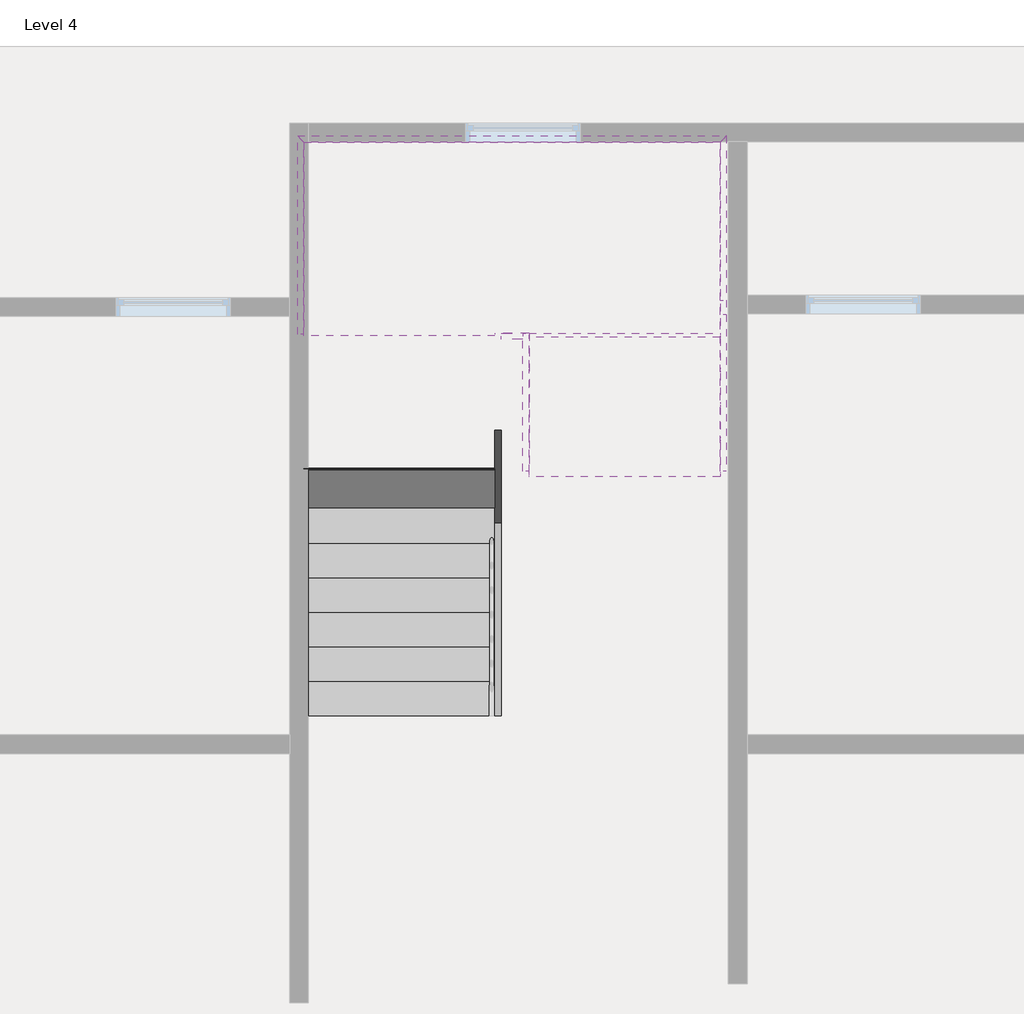
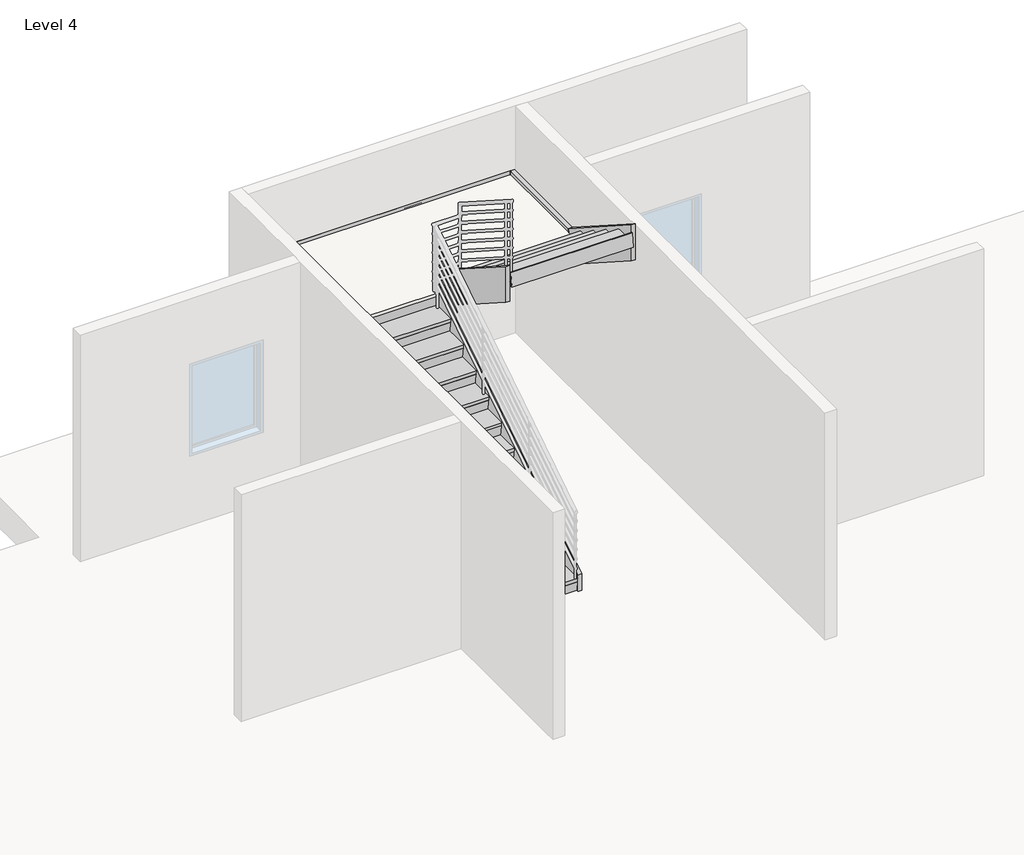
# One storey, part 7 of 7: 8 members, 2 stair flights, 1 slab.
"""IFC4 building model written with IfcOpenShell, lengths in millimetres."""

import ifcopenshell
import ifcopenshell.guid

model = None  # the IFC model being written
_history = None  # IfcOwnerHistory: only IFC2X3 demands one
_inside = {}  # id of a spatial element -> (the spatial element, [elements in it])
_under = {}  # id of a project, library or spatial element -> (it, [spatial elements below it])
_declared = {}  # id of a project -> (the project, [libraries it declares])
_typed = {}  # id of a type object -> (the type object, [elements of that type])
_made_of = {}  # id of a material, layer set ... -> (it, [elements and type objects made of it])


def new_model(schema):
    """Start an empty IFC model of exactly this schema.

    Asked for "IFC4X3", IfcOpenShell would pick the latest addendum, in which some entities
    have other attributes; the version numbers below select the first issue.
    IFC2X3 requires an IfcOwnerHistory on every rooted entity: one is made here for all.
    """
    global model, _history
    if schema == "IFC4X3":
        model = ifcopenshell.file(schema_version=(4, 3, 0, 0))
    else:
        model = ifcopenshell.file(schema=schema)
    _inside.clear()
    _under.clear()
    _declared.clear()
    _typed.clear()
    _made_of.clear()
    _history = None
    if model.schema == "IFC2X3":
        org = make("IfcOrganization", Name="unknown")
        user = make(
            "IfcPersonAndOrganization",
            ThePerson=make("IfcPerson", FamilyName="unknown"),
            TheOrganization=org,
        )
        app = make(
            "IfcApplication",
            ApplicationDeveloper=org,
            Version="unknown",
            ApplicationFullName="unknown",
            ApplicationIdentifier="unknown",
        )
        _history = make(
            "IfcOwnerHistory",
            OwningUser=user,
            OwningApplication=app,
            ChangeAction="ADDED",
            CreationDate=0,
        )
    return model


def make(cls, **values):
    """One entity of the class cls with the attributes given. An attribute that is None is left unset."""
    return model.create_entity(
        cls, **{name: value for name, value in values.items() if value is not None}
    )


def rooted(cls, **values):
    """An entity with a GlobalId (a new one), such as an element, a storey or a relation."""
    return make(cls, GlobalId=ifcopenshell.guid.new(), OwnerHistory=_history, **values)


def si_unit(unit_type, name, prefix=None):
    """IfcSIUnit, for example si_unit("LENGTHUNIT", "METRE", prefix="MILLI")."""
    return make("IfcSIUnit", UnitType=unit_type, Prefix=prefix, Name=name)


def assignment(units):
    """IfcUnitAssignment: the units of a project."""
    return None if units is None else make("IfcUnitAssignment", Units=units)


def point(xyz):
    """IfcCartesianPoint."""
    return None if xyz is None else make("IfcCartesianPoint", Coordinates=xyz)


def direction(xyz):
    """IfcDirection."""
    return None if xyz is None else make("IfcDirection", DirectionRatios=xyz)


def frame(location, z_axis=None, x_axis=None):
    """IfcAxis2Placement3D, a coordinate frame: its origin and axes. An axis left out is left unset."""
    return make(
        "IfcAxis2Placement3D",
        Location=point(location),
        Axis=direction(z_axis),
        RefDirection=direction(x_axis),
    )


def origin():
    """The frame at (0, 0, 0) with its axes left unset."""
    return frame((0.0, 0.0, 0.0))


def place(relative_to, where):
    """IfcLocalPlacement: puts the frame where relative to a parent placement (None: the world)."""
    return make(
        "IfcLocalPlacement", PlacementRelTo=relative_to, RelativePlacement=where
    )


def context(
    kind, dimensions, precision=None, world=None, true_north=None, identifier=None
):
    """IfcGeometricRepresentationContext, for example the 3D "Model" context."""
    return make(
        "IfcGeometricRepresentationContext",
        ContextIdentifier=identifier,
        ContextType=kind,
        CoordinateSpaceDimension=dimensions,
        Precision=precision,
        WorldCoordinateSystem=world,
        TrueNorth=true_north,
    )


def project(units=None, contexts=None):
    """IfcProject with its units and contexts."""
    return rooted(
        "IfcProject",
        Name="project",
        RepresentationContexts=contexts,
        UnitsInContext=assignment(units),
    )


def spatial(cls, under=None, at=None, **own):
    """A site, building, storey or space (cls), placed at a placement, below another one or the project."""
    s = rooted(cls, ObjectPlacement=at, **own)
    if under is not None:
        _under.setdefault(under.id(), (under, []))[1].append(s)
    return s


def polyline(points):
    """IfcPolyline through the points."""
    return make("IfcPolyline", Points=[point(p) for p in points])


def outline(outer, holes=None, kind="AREA"):
    """IfcArbitraryClosedProfileDef: a profile drawn as a closed curve; with holes, ...WithVoids."""
    if holes is None:
        return make("IfcArbitraryClosedProfileDef", ProfileType=kind, OuterCurve=outer)
    return make(
        "IfcArbitraryProfileDefWithVoids",
        ProfileType=kind,
        OuterCurve=outer,
        InnerCurves=holes,
    )


def extrude(swept, where, along, depth):
    """IfcExtrudedAreaSolid: the profile swept, set in the frame where, extruded along a direction by depth."""
    return make(
        "IfcExtrudedAreaSolid",
        SweptArea=swept,
        Position=where,
        ExtrudedDirection=direction(along),
        Depth=depth,
    )


def faces_of(points, faces, orient=None, outer=None):
    """IfcFace entities. A face is a list of loops; a loop is a list of indices into points, from 0.

    orient and outer hold one flag for each loop. By default every Orientation is true, the
    first loop of a face is its IfcFaceOuterBound and the others are IfcFaceBound.
    """
    made = []
    for i, loops in enumerate(faces):
        bounds = []
        for j, loop in enumerate(loops):
            is_outer = j == 0 if outer is None else outer[i][j]
            bounds.append(
                make(
                    "IfcFaceOuterBound" if is_outer else "IfcFaceBound",
                    Bound=make("IfcPolyLoop", Polygon=[points[k] for k in loop]),
                    Orientation=True if orient is None else orient[i][j],
                )
            )
        made.append(make("IfcFace", Bounds=bounds))
    return made


def faceted_brep(points, faces, orient=None, outer=None, voids=None):
    """IfcFacetedBrep: a solid bounded by flat faces; with voids (closed shells), ...WithVoids."""
    shared = [point(p) for p in points]
    hull = make("IfcClosedShell", CfsFaces=faces_of(shared, faces, orient, outer))
    if voids is None:
        return make("IfcFacetedBrep", Outer=hull)
    return make(
        "IfcFacetedBrepWithVoids",
        Outer=hull,
        Voids=[
            make(cls, CfsFaces=faces_of(shared, fs, o, b)) for cls, fs, o, b in voids
        ],
    )


def shape(context_of_items, identifier, shape_type, items):
    """IfcShapeRepresentation: the items that make up one representation, for example the "Body"."""
    return make(
        "IfcShapeRepresentation",
        ContextOfItems=context_of_items,
        RepresentationIdentifier=identifier,
        RepresentationType=shape_type,
        Items=items,
    )


def source(mapping_origin, context_of_items, identifier, shape_type, items):
    """IfcRepresentationMap: a shape defined once, which mapped items show again and again."""
    return make(
        "IfcRepresentationMap",
        MappingOrigin=mapping_origin,
        MappedRepresentation=shape(context_of_items, identifier, shape_type, items),
    )


def transform(
    local_origin,
    x_axis=None,
    y_axis=None,
    z_axis=None,
    scale=None,
    scale2=None,
    scale3=None,
    uniform=True,
):
    """IfcCartesianTransformationOperator3D, or its non-uniform kind. x_axis, y_axis, z_axis: its Axis1, 2, 3."""
    if uniform:
        return make(
            "IfcCartesianTransformationOperator3D",
            Axis1=direction(x_axis),
            Axis2=direction(y_axis),
            LocalOrigin=point(local_origin),
            Scale=scale,
            Axis3=direction(z_axis),
        )
    return make(
        "IfcCartesianTransformationOperator3DnonUniform",
        Axis1=direction(x_axis),
        Axis2=direction(y_axis),
        LocalOrigin=point(local_origin),
        Scale=scale,
        Axis3=direction(z_axis),
        Scale2=scale2,
        Scale3=scale3,
    )


def mapped(mapping_source, mapping_target):
    """IfcMappedItem: shows the shape of a source again, moved by a transform."""
    return make(
        "IfcMappedItem", MappingSource=mapping_source, MappingTarget=mapping_target
    )


def made_of(thing, what):
    """Note that an element or type object is made of a material, layer set ...; save() writes the relation."""
    if what is not None:
        _made_of.setdefault(what.id(), (what, []))[1].append(thing)
    return thing


def element(
    cls,
    number,
    at=None,
    inside=None,
    cuts=None,
    type_object=None,
    material=None,
    context=None,
    identifier="Body",
    shape_type=None,
    held_by="IfcProductDefinitionShape",
    body=None,
    shapes=None,
    **own,
):
    """One element of the class cls, such as IfcWall. Its Tag is "e" and its number.

    at: its placement. inside: the storey or other place that contains it. cuts: it is an
    opening in that element (IfcRelVoidsElement). A single representation is given by context,
    identifier, shape_type and body (its items); several are given by shapes. held_by: the class
    of the entity that holds the representations. save() writes the other relations.
    """
    e = rooted(cls, Tag="e%d" % number, ObjectPlacement=at, **own)
    if body is not None:
        shapes = [shape(context, identifier, shape_type, body)]
    if shapes is not None:
        e.Representation = make(held_by, Representations=shapes)
    if inside is not None:
        _inside.setdefault(inside.id(), (inside, []))[1].append(e)
    if cuts is not None:
        rooted(
            "IfcRelVoidsElement", RelatingBuildingElement=cuts, RelatedOpeningElement=e
        )
    if type_object is not None:
        _typed.setdefault(type_object.id(), (type_object, []))[1].append(e)
    return made_of(e, material)


def aggregate(whole, parts):
    """IfcRelAggregates: a whole, such as a stair, and the parts it consists of."""
    return rooted("IfcRelAggregates", RelatingObject=whole, RelatedObjects=parts)


def save(model, path):
    """Write the relations noted so far, then the file.

    IfcRelAggregates (storeys below a building ...), IfcRelContainedInSpatialStructure (elements
    in a storey), IfcRelDefinesByType, IfcRelAssociatesMaterial and IfcRelDeclares: one each for
    every whole, place, type object, material and project.
    """
    for whole, parts in _under.values():
        aggregate(whole, parts)
    for where, things in _inside.values():
        rooted(
            "IfcRelContainedInSpatialStructure",
            RelatedElements=things,
            RelatingStructure=where,
        )
    for kind, things in _typed.values():
        rooted("IfcRelDefinesByType", RelatedObjects=things, RelatingType=kind)
    for what, things in _made_of.values():
        rooted("IfcRelAssociatesMaterial", RelatedObjects=things, RelatingMaterial=what)
    for by, libraries in _declared.values():
        rooted("IfcRelDeclares", RelatingContext=by, RelatedDefinitions=libraries)
    model.write(path)


def non_monolithic_landing_893569eb(model_context):
    return source(origin(), model_context, "Body", "Brep", [
        faceted_brep([(-226.7120949, 7307.4781803, 11617.6470588), (-226.7120949, 7300.3948469, 11567.6470588), (1293.2879051, 7300.3948469, 11567.6470588), (1293.2879051, 7307.4781803, 11617.6470588), (-499.4393676, 7309.7509075, 11617.6470588), (-499.4393676, 7332.4781803, 11617.6470588), (-226.7120949, 7332.4781803, 11617.6470588), (1293.2879051, 7332.4781803, 11617.6470588), (1293.2879051, 8852.4781803, 11617.6470588), (-2019.4393676, 8852.4781803, 11617.6470588), (-2019.4393676, 7309.7509075, 11617.6470588), (-226.7120949, 7332.4781803, 11567.6470588), (-499.4393676, 7332.4781803, 11567.6470588), (-499.4393676, 7316.8342409, 11567.6470588), (-2019.4393676, 7316.8342409, 11567.6470588), (-2019.4393676, 8852.4781803, 11567.6470588), (1293.2879051, 8852.4781803, 11567.6470588), (1293.2879051, 7332.4781803, 11567.6470588)], [[[0, 1, 2, 3]], [[4, 5, 6, 0, 3, 7, 8, 9, 10]], [[11, 12, 13, 14, 15, 16, 17, 2, 1]], [[5, 4, 13, 12]], [[6, 5, 12, 11]], [[0, 6, 11, 1]], [[7, 3, 2, 17]], [[8, 7, 17, 16]], [[9, 8, 16, 15]], [[10, 9, 15, 14]], [[4, 10, 14, 13]]]),
    ])


def stair_flight_50mm_tread_25mm_nosing_13mm_riser_ea8afa7a(model_context):
    return source(origin(), model_context, "Body", "Brep", [
        faceted_brep([(-499.4393676, 4584.7509075, 9676.4705882), (-499.4393676, 4591.8342409, 9626.4705882), (-2019.4393676, 4591.8342409, 9626.4705882), (-2019.4393676, 4584.7509075, 9676.4705882), (-2019.4393676, 4284.7509075, 9676.4705882), (-499.4393676, 4284.7509075, 9676.4705882), (-499.4393676, 4291.8342409, 9626.4705882), (-2019.4393676, 4291.8342409, 9626.4705882)], [[[0, 1, 2, 3]], [[3, 4, 5, 0]], [[2, 1, 6, 7]], [[4, 3, 2, 7]], [[0, 5, 6, 1]], [[5, 4, 7, 6]]]),
        faceted_brep([(-499.4393676, 4291.8342409, 9626.4705882), (-499.4393676, 4309.7509075, 9500.0), (-499.4393676, 4322.3757185, 9500.0), (-499.4393676, 4304.4590518, 9626.4705882), (-2019.4393676, 4291.8342409, 9626.4705882), (-2019.4393676, 4304.4590518, 9626.4705882), (-2019.4393676, 4322.3757185, 9500.0), (-2019.4393676, 4309.7509075, 9500.0)], [[[0, 1, 2, 3]], [[4, 5, 6, 7]], [[1, 0, 4, 7]], [[2, 1, 7, 6]], [[3, 2, 6, 5]], [[0, 3, 5, 4]]]),
        faceted_brep([(-499.4393676, 4566.8342409, 9802.9411765), (-499.4393676, 4591.8342409, 9626.4705882), (-499.4393676, 4604.4590518, 9626.4705882), (-499.4393676, 4579.4590518, 9802.9411765), (-2019.4393676, 4566.8342409, 9802.9411765), (-2019.4393676, 4579.4590518, 9802.9411765), (-2019.4393676, 4604.4590518, 9626.4705882), (-2019.4393676, 4591.8342409, 9626.4705882)], [[[0, 1, 2, 3]], [[4, 5, 6, 7]], [[1, 0, 4, 7]], [[2, 1, 7, 6]], [[3, 2, 6, 5]], [[0, 3, 5, 4]]]),
        faceted_brep([(-2019.4393676, 4859.7509075, 9852.9411765), (-2019.4393676, 4559.7509075, 9852.9411765), (-499.4393676, 4559.7509075, 9852.9411765), (-499.4393676, 4859.7509075, 9852.9411765), (-2019.4393676, 4866.8342409, 9802.9411765), (-499.4393676, 4866.8342409, 9802.9411765), (-499.4393676, 4566.8342409, 9802.9411765), (-2019.4393676, 4566.8342409, 9802.9411765)], [[[0, 1, 2, 3]], [[4, 5, 6, 7]], [[1, 0, 4, 7]], [[3, 2, 6, 5]], [[3, 5, 4, 0]], [[2, 1, 7, 6]]]),
        faceted_brep([(-499.4393676, 4841.8342409, 9979.4117647), (-499.4393676, 4866.8342409, 9802.9411765), (-499.4393676, 4879.4590518, 9802.9411765), (-499.4393676, 4854.4590518, 9979.4117647), (-2019.4393676, 4841.8342409, 9979.4117647), (-2019.4393676, 4854.4590518, 9979.4117647), (-2019.4393676, 4879.4590518, 9802.9411765), (-2019.4393676, 4866.8342409, 9802.9411765)], [[[0, 1, 2, 3]], [[4, 5, 6, 7]], [[1, 0, 4, 7]], [[2, 1, 7, 6]], [[3, 2, 6, 5]], [[0, 3, 5, 4]]]),
        faceted_brep([(-2019.4393676, 5134.7509075, 10029.4117647), (-2019.4393676, 4834.7509075, 10029.4117647), (-499.4393676, 4834.7509075, 10029.4117647), (-499.4393676, 5134.7509075, 10029.4117647), (-2019.4393676, 5141.8342409, 9979.4117647), (-499.4393676, 5141.8342409, 9979.4117647), (-499.4393676, 4841.8342409, 9979.4117647), (-2019.4393676, 4841.8342409, 9979.4117647)], [[[0, 1, 2, 3]], [[4, 5, 6, 7]], [[1, 0, 4, 7]], [[3, 2, 6, 5]], [[3, 5, 4, 0]], [[2, 1, 7, 6]]]),
        faceted_brep([(-499.4393676, 5116.8342409, 10155.8823529), (-499.4393676, 5141.8342409, 9979.4117647), (-499.4393676, 5154.4590518, 9979.4117647), (-499.4393676, 5129.4590518, 10155.8823529), (-2019.4393676, 5116.8342409, 10155.8823529), (-2019.4393676, 5129.4590518, 10155.8823529), (-2019.4393676, 5154.4590518, 9979.4117647), (-2019.4393676, 5141.8342409, 9979.4117647)], [[[0, 1, 2, 3]], [[4, 5, 6, 7]], [[1, 0, 4, 7]], [[2, 1, 7, 6]], [[3, 2, 6, 5]], [[0, 3, 5, 4]]]),
        faceted_brep([(-2019.4393676, 5409.7509075, 10205.8823529), (-2019.4393676, 5109.7509075, 10205.8823529), (-499.4393676, 5109.7509075, 10205.8823529), (-499.4393676, 5409.7509075, 10205.8823529), (-2019.4393676, 5416.8342409, 10155.8823529), (-499.4393676, 5416.8342409, 10155.8823529), (-499.4393676, 5116.8342409, 10155.8823529), (-2019.4393676, 5116.8342409, 10155.8823529)], [[[0, 1, 2, 3]], [[4, 5, 6, 7]], [[1, 0, 4, 7]], [[3, 2, 6, 5]], [[3, 5, 4, 0]], [[2, 1, 7, 6]]]),
        faceted_brep([(-499.4393676, 5391.8342409, 10332.3529412), (-499.4393676, 5416.8342409, 10155.8823529), (-499.4393676, 5429.4590518, 10155.8823529), (-499.4393676, 5404.4590518, 10332.3529412), (-2019.4393676, 5391.8342409, 10332.3529412), (-2019.4393676, 5404.4590518, 10332.3529412), (-2019.4393676, 5429.4590518, 10155.8823529), (-2019.4393676, 5416.8342409, 10155.8823529)], [[[0, 1, 2, 3]], [[4, 5, 6, 7]], [[1, 0, 4, 7]], [[2, 1, 7, 6]], [[3, 2, 6, 5]], [[0, 3, 5, 4]]]),
        faceted_brep([(-2019.4393676, 5684.7509075, 10382.3529412), (-2019.4393676, 5384.7509075, 10382.3529412), (-499.4393676, 5384.7509075, 10382.3529412), (-499.4393676, 5684.7509075, 10382.3529412), (-2019.4393676, 5691.8342409, 10332.3529412), (-499.4393676, 5691.8342409, 10332.3529412), (-499.4393676, 5391.8342409, 10332.3529412), (-2019.4393676, 5391.8342409, 10332.3529412)], [[[0, 1, 2, 3]], [[4, 5, 6, 7]], [[1, 0, 4, 7]], [[3, 2, 6, 5]], [[3, 5, 4, 0]], [[2, 1, 7, 6]]]),
        faceted_brep([(-499.4393676, 5666.8342409, 10508.8235294), (-499.4393676, 5691.8342409, 10332.3529412), (-499.4393676, 5704.4590518, 10332.3529412), (-499.4393676, 5679.4590518, 10508.8235294), (-2019.4393676, 5666.8342409, 10508.8235294), (-2019.4393676, 5679.4590518, 10508.8235294), (-2019.4393676, 5704.4590518, 10332.3529412), (-2019.4393676, 5691.8342409, 10332.3529412)], [[[0, 1, 2, 3]], [[4, 5, 6, 7]], [[1, 0, 4, 7]], [[2, 1, 7, 6]], [[3, 2, 6, 5]], [[0, 3, 5, 4]]]),
        faceted_brep([(-2019.4393676, 5959.7509075, 10558.8235294), (-2019.4393676, 5659.7509075, 10558.8235294), (-499.4393676, 5659.7509075, 10558.8235294), (-499.4393676, 5959.7509075, 10558.8235294), (-2019.4393676, 5966.8342409, 10508.8235294), (-499.4393676, 5966.8342409, 10508.8235294), (-499.4393676, 5666.8342409, 10508.8235294), (-2019.4393676, 5666.8342409, 10508.8235294)], [[[0, 1, 2, 3]], [[4, 5, 6, 7]], [[1, 0, 4, 7]], [[3, 2, 6, 5]], [[3, 5, 4, 0]], [[2, 1, 7, 6]]]),
        faceted_brep([(-499.4393676, 5941.8342409, 10685.2941176), (-499.4393676, 5966.8342409, 10508.8235294), (-499.4393676, 5979.4590518, 10508.8235294), (-499.4393676, 5954.4590518, 10685.2941176), (-2019.4393676, 5941.8342409, 10685.2941176), (-2019.4393676, 5954.4590518, 10685.2941176), (-2019.4393676, 5979.4590518, 10508.8235294), (-2019.4393676, 5966.8342409, 10508.8235294)], [[[0, 1, 2, 3]], [[4, 5, 6, 7]], [[1, 0, 4, 7]], [[2, 1, 7, 6]], [[3, 2, 6, 5]], [[0, 3, 5, 4]]]),
        faceted_brep([(-2019.4393676, 6234.7509075, 10735.2941176), (-2019.4393676, 5934.7509075, 10735.2941176), (-499.4393676, 5934.7509075, 10735.2941176), (-499.4393676, 6234.7509075, 10735.2941176), (-2019.4393676, 6241.8342409, 10685.2941176), (-499.4393676, 6241.8342409, 10685.2941176), (-499.4393676, 5941.8342409, 10685.2941176), (-2019.4393676, 5941.8342409, 10685.2941176)], [[[0, 1, 2, 3]], [[4, 5, 6, 7]], [[1, 0, 4, 7]], [[3, 2, 6, 5]], [[3, 5, 4, 0]], [[2, 1, 7, 6]]]),
        faceted_brep([(-499.4393676, 6216.8342409, 10861.7647059), (-499.4393676, 6241.8342409, 10685.2941176), (-499.4393676, 6254.4590518, 10685.2941176), (-499.4393676, 6229.4590518, 10861.7647059), (-2019.4393676, 6216.8342409, 10861.7647059), (-2019.4393676, 6229.4590518, 10861.7647059), (-2019.4393676, 6254.4590518, 10685.2941176), (-2019.4393676, 6241.8342409, 10685.2941176)], [[[0, 1, 2, 3]], [[4, 5, 6, 7]], [[1, 0, 4, 7]], [[2, 1, 7, 6]], [[3, 2, 6, 5]], [[0, 3, 5, 4]]]),
        faceted_brep([(-2019.4393676, 6509.7509075, 10911.7647059), (-2019.4393676, 6209.7509075, 10911.7647059), (-499.4393676, 6209.7509075, 10911.7647059), (-499.4393676, 6509.7509075, 10911.7647059), (-2019.4393676, 6516.8342409, 10861.7647059), (-499.4393676, 6516.8342409, 10861.7647059), (-499.4393676, 6216.8342409, 10861.7647059), (-2019.4393676, 6216.8342409, 10861.7647059)], [[[0, 1, 2, 3]], [[4, 5, 6, 7]], [[1, 0, 4, 7]], [[3, 2, 6, 5]], [[3, 5, 4, 0]], [[2, 1, 7, 6]]]),
        faceted_brep([(-499.4393676, 6491.8342409, 11038.2352941), (-499.4393676, 6516.8342409, 10861.7647059), (-499.4393676, 6529.4590518, 10861.7647059), (-499.4393676, 6504.4590518, 11038.2352941), (-2019.4393676, 6491.8342409, 11038.2352941), (-2019.4393676, 6504.4590518, 11038.2352941), (-2019.4393676, 6529.4590518, 10861.7647059), (-2019.4393676, 6516.8342409, 10861.7647059)], [[[0, 1, 2, 3]], [[4, 5, 6, 7]], [[1, 0, 4, 7]], [[2, 1, 7, 6]], [[3, 2, 6, 5]], [[0, 3, 5, 4]]]),
        faceted_brep([(-2019.4393676, 6784.7509075, 11088.2352941), (-2019.4393676, 6484.7509075, 11088.2352941), (-499.4393676, 6484.7509075, 11088.2352941), (-499.4393676, 6784.7509075, 11088.2352941), (-2019.4393676, 6791.8342409, 11038.2352941), (-499.4393676, 6791.8342409, 11038.2352941), (-499.4393676, 6491.8342409, 11038.2352941), (-2019.4393676, 6491.8342409, 11038.2352941)], [[[0, 1, 2, 3]], [[4, 5, 6, 7]], [[1, 0, 4, 7]], [[3, 2, 6, 5]], [[3, 5, 4, 0]], [[2, 1, 7, 6]]]),
        faceted_brep([(-499.4393676, 6766.8342409, 11214.7058824), (-499.4393676, 6791.8342409, 11038.2352941), (-499.4393676, 6804.4590518, 11038.2352941), (-499.4393676, 6779.4590518, 11214.7058824), (-2019.4393676, 6766.8342409, 11214.7058824), (-2019.4393676, 6779.4590518, 11214.7058824), (-2019.4393676, 6804.4590518, 11038.2352941), (-2019.4393676, 6791.8342409, 11038.2352941)], [[[0, 1, 2, 3]], [[4, 5, 6, 7]], [[1, 0, 4, 7]], [[2, 1, 7, 6]], [[3, 2, 6, 5]], [[0, 3, 5, 4]]]),
        faceted_brep([(-2019.4393676, 7059.7509075, 11264.7058824), (-2019.4393676, 6759.7509075, 11264.7058824), (-499.4393676, 6759.7509075, 11264.7058824), (-499.4393676, 7059.7509075, 11264.7058824), (-2019.4393676, 7066.8342409, 11214.7058824), (-499.4393676, 7066.8342409, 11214.7058824), (-499.4393676, 6766.8342409, 11214.7058824), (-2019.4393676, 6766.8342409, 11214.7058824)], [[[0, 1, 2, 3]], [[4, 5, 6, 7]], [[1, 0, 4, 7]], [[3, 2, 6, 5]], [[3, 5, 4, 0]], [[2, 1, 7, 6]]]),
        faceted_brep([(-499.4393676, 7316.8342409, 11567.6470588), (-499.4393676, 7341.8342409, 11391.1764706), (-499.4393676, 7354.4590518, 11391.1764706), (-499.4393676, 7329.4590518, 11567.6470588), (-2019.4393676, 7316.8342409, 11567.6470588), (-2019.4393676, 7329.4590518, 11567.6470588), (-2019.4393676, 7354.4590518, 11391.1764706), (-2019.4393676, 7341.8342409, 11391.1764706)], [[[0, 1, 2, 3]], [[4, 5, 6, 7]], [[1, 0, 4, 7]], [[2, 1, 7, 6]], [[3, 2, 6, 5]], [[0, 3, 5, 4]]]),
        faceted_brep([(-499.4393676, 7041.8342409, 11391.1764706), (-499.4393676, 7066.8342409, 11214.7058824), (-499.4393676, 7079.4590518, 11214.7058824), (-499.4393676, 7054.4590518, 11391.1764706), (-2019.4393676, 7041.8342409, 11391.1764706), (-2019.4393676, 7054.4590518, 11391.1764706), (-2019.4393676, 7079.4590518, 11214.7058824), (-2019.4393676, 7066.8342409, 11214.7058824)], [[[0, 1, 2, 3]], [[4, 5, 6, 7]], [[1, 0, 4, 7]], [[2, 1, 7, 6]], [[3, 2, 6, 5]], [[0, 3, 5, 4]]]),
        faceted_brep([(-2019.4393676, 7334.7509075, 11441.1764706), (-2019.4393676, 7309.7509075, 11441.1764706), (-2019.4393676, 7034.7509075, 11441.1764706), (-499.4393676, 7034.7509075, 11441.1764706), (-499.4393676, 7334.7509075, 11441.1764706), (-2019.4393676, 7341.8342409, 11391.1764706), (-499.4393676, 7341.8342409, 11391.1764706), (-499.4393676, 7041.8342409, 11391.1764706), (-2019.4393676, 7041.8342409, 11391.1764706), (-2019.4393676, 7309.7509075, 11391.1764706)], [[[0, 1, 2, 3, 4]], [[5, 6, 7, 8, 9]], [[1, 0, 5, 9]], [[2, 1, 9, 8]], [[4, 3, 7, 6]], [[4, 6, 5, 0]], [[3, 2, 8, 7]]]),
    ])


def stair_flight_50mm_tread_25mm_nosing_13mm_riser_c8de7c0f(model_context):
    return source(origin(), model_context, "Body", "SweptSolid", [
        extrude(outline(polyline([(7032.4781803, 11794.1176471), (7332.4781803, 11794.1176471), (7325.3948469, 11744.1176471), (7025.3948469, 11744.1176471), (7032.4781803, 11794.1176471)])), frame((-226.7120949, 0.0, 0.0), z_axis=(1.0, 0.0, 0.0), x_axis=(0.0, 1.0, 0.0)), (0.0, 0.0, 1.0), 1520.0),
        extrude(outline(polyline([(7325.3948469, 11744.1176471), (7300.3948469, 11567.6470588), (7287.770036, 11567.6470588), (7312.770036, 11744.1176471), (7325.3948469, 11744.1176471)])), frame((-226.7120949, 0.0, 0.0), z_axis=(1.0, 0.0, 0.0), x_axis=(0.0, 1.0, 0.0)), (0.0, 0.0, 1.0), 1520.0),
        extrude(outline(polyline([(7050.3948469, 11920.5882353), (7025.3948469, 11744.1176471), (7012.770036, 11744.1176471), (7037.770036, 11920.5882353), (7050.3948469, 11920.5882353)])), frame((-226.7120949, 0.0, 0.0), z_axis=(1.0, 0.0, 0.0), x_axis=(0.0, 1.0, 0.0)), (0.0, 0.0, 1.0), 1520.0),
        extrude(outline(polyline([(6757.4781803, 11970.5882353), (7057.4781803, 11970.5882353), (7050.3948469, 11920.5882353), (6750.3948469, 11920.5882353), (6757.4781803, 11970.5882353)])), frame((-226.7120949, 0.0, 0.0), z_axis=(1.0, 0.0, 0.0), x_axis=(0.0, 1.0, 0.0)), (0.0, 0.0, 1.0), 1520.0),
        extrude(outline(polyline([(6775.3948469, 12097.0588235), (6750.3948469, 11920.5882353), (6737.770036, 11920.5882353), (6762.770036, 12097.0588235), (6775.3948469, 12097.0588235)])), frame((-226.7120949, 0.0, 0.0), z_axis=(1.0, 0.0, 0.0), x_axis=(0.0, 1.0, 0.0)), (0.0, 0.0, 1.0), 1520.0),
        extrude(outline(polyline([(6482.4781803, 12147.0588235), (6782.4781803, 12147.0588235), (6775.3948469, 12097.0588235), (6475.3948469, 12097.0588235), (6482.4781803, 12147.0588235)])), frame((-226.7120949, 0.0, 0.0), z_axis=(1.0, 0.0, 0.0), x_axis=(0.0, 1.0, 0.0)), (0.0, 0.0, 1.0), 1520.0),
        extrude(outline(polyline([(6500.3948469, 12273.5294118), (6475.3948469, 12097.0588235), (6462.770036, 12097.0588235), (6487.770036, 12273.5294118), (6500.3948469, 12273.5294118)])), frame((-226.7120949, 0.0, 0.0), z_axis=(1.0, 0.0, 0.0), x_axis=(0.0, 1.0, 0.0)), (0.0, 0.0, 1.0), 1520.0),
        extrude(outline(polyline([(6225.3948469, 12450.0), (6200.3948469, 12273.5294118), (6187.770036, 12273.5294118), (6212.770036, 12450.0), (6225.3948469, 12450.0)])), frame((-226.7120949, 0.0, 0.0), z_axis=(1.0, 0.0, 0.0), x_axis=(0.0, 1.0, 0.0)), (0.0, 0.0, 1.0), 1520.0),
        extrude(outline(polyline([(6207.4781803, 12323.5294118), (6507.4781803, 12323.5294118), (6500.3948469, 12273.5294118), (6200.3948469, 12273.5294118), (6207.4781803, 12323.5294118)])), frame((-226.7120949, 0.0, 0.0), z_axis=(1.0, 0.0, 0.0), x_axis=(0.0, 1.0, 0.0)), (0.0, 0.0, 1.0), 1520.0),
    ])


model = new_model("IFC4")

# Units and contexts
model_context = context("Model", 3, world=origin())
ifc_project = project(units=[si_unit("LENGTHUNIT", "METRE", prefix="MILLI")], contexts=[model_context])

# Site, building, storey
site = spatial("IfcSite", under=ifc_project)
building = spatial("IfcBuilding", under=site)
storey = spatial("IfcBuildingStorey", under=building, Name="Level 4", Elevation=9500.0)

# Members
placement = place(None, origin())
element("IfcMember", 1, ObjectType="Stringer - 50mm Width", at=placement, inside=storey, context=model_context, shape_type="SweptSolid", body=[
    extrude(outline(polyline([(4284.7509075, 9500.0), (4284.7509075, 9715.9811749), (7322.0354678, 11665.0407858), (7439.3399977, 11265.0407858), (4688.8181065, 9500.0), (4284.7509075, 9500.0)])), frame((-2069.4393676, 0.0, 0.0), z_axis=(1.0, 0.0, 0.0), x_axis=(0.0, 1.0, 0.0)), (0.0, 0.0, 1.0), 50.0),
])
element("IfcMember", 2, ObjectType="Stringer - 50mm Width", at=placement, inside=storey, context=model_context, shape_type="SweptSolid", body=[
    extrude(outline(polyline([(4284.7509075, 9500.0), (4284.7509075, 9715.9811749), (7322.0354678, 11665.0407858), (7332.4781803, 11665.0407858), (7332.4781803, 11196.4663575), (4688.8181065, 9500.0), (4284.7509075, 9500.0)])), frame((-499.4393676, 0.0, 0.0), z_axis=(1.0, 0.0, 0.0), x_axis=(0.0, 1.0, 0.0)), (0.0, 0.0, 1.0), 50.0),
])
element("IfcMember", 3, ObjectType="Stringer - 50mm Width", at=placement, inside=storey, context=model_context, shape_type="SweptSolid", body=[
    extrude(outline(polyline([(7595.19362, 11665.0407858), (7477.8890902, 11265.0407858), (6232.4781803, 12064.2349525), (6232.4781803, 12539.5105867), (7595.19362, 11665.0407858)])), frame((1293.2879051, 0.0, 0.0), z_axis=(1.0, 0.0, 0.0), x_axis=(0.0, 1.0, 0.0)), (0.0, 0.0, 1.0), 50.0),
])
element("IfcMember", 4, ObjectType="Stringer - 50mm Width", at=placement, inside=storey, context=model_context, shape_type="SweptSolid", body=[
    extrude(outline(polyline([(7332.4781803, 11833.6282338), (7332.4781803, 11358.3525996), (6232.4781803, 12064.2349525), (6232.4781803, 12539.5105867), (7332.4781803, 11833.6282338)])), frame((-276.7120949, 0.0, 0.0), z_axis=(1.0, 0.0, 0.0), x_axis=(0.0, 1.0, 0.0)), (0.0, 0.0, 1.0), 50.0),
])
element("IfcMember", 5, ObjectType="Stringer - 50mm Width", at=placement, inside=storey, context=model_context, shape_type="Brep", body=[
    faceted_brep([(1293.2879051, 7595.19362, 11665.0407858), (1343.2879051, 7595.19362, 11665.0407858), (1343.2879051, 8902.4781803, 11665.0407858), (1293.2879051, 8852.4781803, 11665.0407858), (1293.2879051, 7477.8890902, 11265.0407858), (1293.2879051, 8852.4781803, 11265.0407858), (1343.2879051, 7477.8890902, 11265.0407858), (1343.2879051, 8902.4781803, 11265.0407858)], [[[0, 1, 2, 3]], [[4, 0, 3, 5]], [[6, 4, 5, 7]], [[1, 6, 7, 2]], [[1, 0, 4, 6]], [[2, 7, 5, 3]]]),
])
element("IfcMember", 6, ObjectType="Stringer - 50mm Width", at=placement, inside=storey, context=model_context, shape_type="SweptSolid", body=[
    extrude(outline(polyline([(1343.2879051, 8902.4781803), (1293.2879051, 8852.4781803), (-2019.4393676, 8852.4781803), (-2069.4393676, 8902.4781803), (1343.2879051, 8902.4781803)])), frame((0.0, 0.0, 11265.0407858), z_axis=(0.0, 0.0, 1.0), x_axis=(1.0, 0.0, 0.0)), (0.0, 0.0, 1.0), 400.0),
])
element("IfcMember", 7, ObjectType="Stringer - 50mm Width", at=placement, inside=storey, context=model_context, shape_type="Brep", body=[
    faceted_brep([(-2019.4393676, 8852.4781803, 11665.0407858), (-2069.4393676, 8902.4781803, 11665.0407858), (-2069.4393676, 7322.0354678, 11665.0407858), (-2019.4393676, 7322.0354678, 11665.0407858), (-2019.4393676, 8852.4781803, 11265.0407858), (-2019.4393676, 7439.3399977, 11265.0407858), (-2069.4393676, 8902.4781803, 11265.0407858), (-2069.4393676, 7439.3399977, 11265.0407858)], [[[0, 1, 2, 3]], [[4, 0, 3, 5]], [[6, 4, 5, 7]], [[1, 6, 7, 2]], [[1, 0, 4, 6]], [[2, 7, 5, 3]]]),
])
element("IfcMember", 8, ObjectType="Stringer - 50mm Width", at=placement, inside=storey, context=model_context, shape_type="SweptSolid", body=[
    extrude(outline(polyline([(-449.4393676, 7282.4781803), (-449.4393676, 7332.4781803), (-276.7120949, 7332.4781803), (-276.7120949, 7282.4781803), (-449.4393676, 7282.4781803)])), frame((0.0, 0.0, 11265.0407858), z_axis=(0.0, 0.0, 1.0), x_axis=(1.0, 0.0, 0.0)), (0.0, 0.0, 1.0), 400.0),
])

# Slab
non_monolithic_landing_shape = non_monolithic_landing_893569eb(model_context)
element("IfcSlab", 9, ObjectType="Non-Monolithic Landing", at=placement, inside=storey, context=model_context, shape_type="MappedRepresentation", body=[
    mapped(non_monolithic_landing_shape, transform((0.0, 0.0, 0.0), x_axis=(1.0, 0.0, 0.0), y_axis=(0.0, 1.0, 0.0), z_axis=(0.0, 0.0, 1.0))),
])

# Stair flights
stair_flight_50mm_tread_25mm_nosing_13mm_riser_shape = stair_flight_50mm_tread_25mm_nosing_13mm_riser_ea8afa7a(model_context)
element("IfcStairFlight", 10, ObjectType="50mm Tread 25mm Nosing 13mm Riser", at=placement, inside=storey, context=model_context, shape_type="MappedRepresentation", body=[
    mapped(stair_flight_50mm_tread_25mm_nosing_13mm_riser_shape, transform((0.0, 0.0, 0.0), x_axis=(1.0, 0.0, 0.0), y_axis=(0.0, 1.0, 0.0), z_axis=(0.0, 0.0, 1.0))),
])
stair_flight_50mm_tread_25mm_nosing_13mm_riser_2_shape = stair_flight_50mm_tread_25mm_nosing_13mm_riser_c8de7c0f(model_context)
element("IfcStairFlight", 11, ObjectType="50mm Tread 25mm Nosing 13mm Riser", at=placement, inside=storey, context=model_context, shape_type="MappedRepresentation", body=[
    mapped(stair_flight_50mm_tread_25mm_nosing_13mm_riser_2_shape, transform((0.0, 0.0, 0.0), x_axis=(1.0, 0.0, 0.0), y_axis=(0.0, 1.0, 0.0), z_axis=(0.0, 0.0, 1.0))),
])

save(model, "model.ifc")

# Revit data of these elements
# Elements 1, 2, 3, 4, 5, 6, 7, 8 (IfcMember, "Stringer - 50mm Width")
#   Phase Created = New Construction
# Element 9 (IfcSlab, "Non-Monolithic Landing")
#   Phase Created = New Construction
# Elements 10, 11 (IfcStairFlight, "50mm Tread 25mm Nosing 13mm Riser")
#   Phase Created = New Construction
